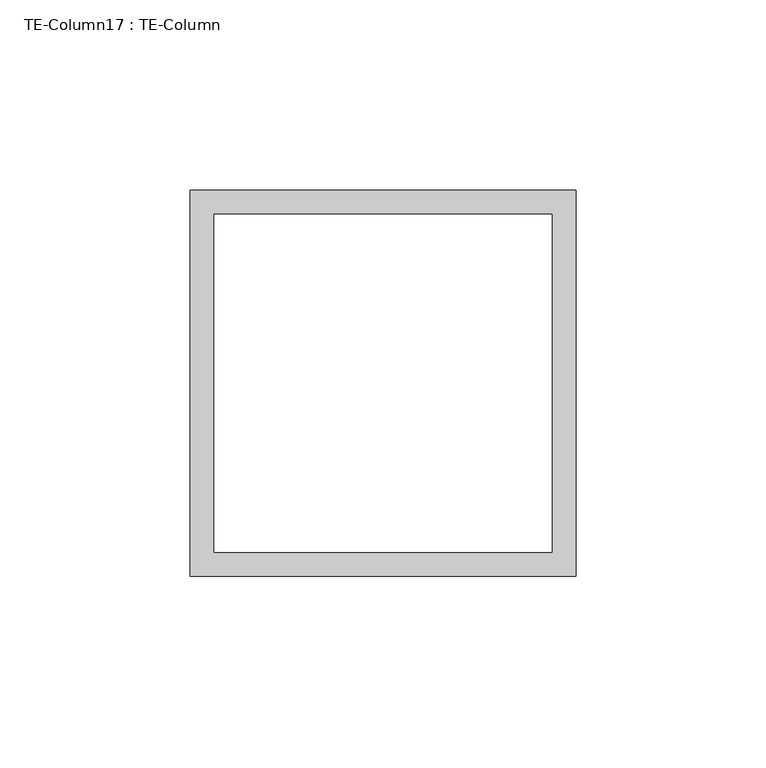
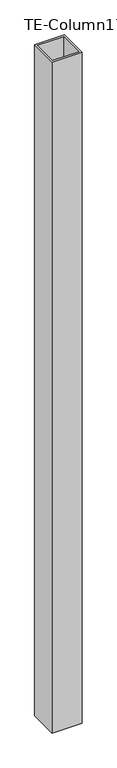
"""IFC4 building model written with IfcOpenShell, lengths in millimetres: proxy geometry, TE-Column17 : TE-Column."""

from ifc_helpers import new_model, si_unit, frame, origin, place, context, project, spatial, polyline, outline, extrude, source, transform, mapped, element, save


def te_column17_te_column_a47af242(model_context):
    return source(origin(), model_context, "Body", "SweptSolid", [
        extrude(outline(polyline([(590318.6434739, -536417.5913841), (590217.0434739, -536417.5913841), (590217.0434739, -536315.9913841), (590318.6434739, -536315.9913841), (590318.6434739, -536417.5913841)]), holes=[polyline([(590312.2934739, -536322.3413841), (590223.3934739, -536322.3413841), (590223.3934739, -536411.2413841), (590312.2934739, -536411.2413841), (590312.2934739, -536322.3413841)])]), frame((0.0, 0.0, 28.575), z_axis=(0.0, 0.0, 1.0), x_axis=(1.0, 0.0, 0.0)), (0.0, 0.0, 1.0), 2406.65),
    ])


if __name__ == "__main__":
    model = new_model("IFC4")
    model_context = context("Model", 3, world=origin())
    ifc_project = project(units=[si_unit("LENGTHUNIT", "METRE", prefix="MILLI")], contexts=[model_context])
    site = spatial("IfcSite", under=ifc_project)
    building = spatial("IfcBuilding", under=site)
    placement = place(None, origin())
    te_column17_te_column_shape = te_column17_te_column_a47af242(model_context)
    element("IfcBuildingElementProxy", 1, Name="TE-Column17 : TE-Column", ObjectType="TE-Column17 : TE-Column", at=placement, inside=building, context=model_context, shape_type="MappedRepresentation", body=[
        mapped(te_column17_te_column_shape, transform((0.0, 0.0, 0.0), x_axis=(1.0, 0.0, 0.0), y_axis=(0.0, 1.0, 0.0), z_axis=(0.0, 0.0, 1.0))),
    ])
    save(model, "model.ifc")

# Revit data of these elements
# Element 1 (IfcBuildingElementProxy, "TE-Column17 : TE-Column")
#   Materials on its faces: "4\"X4\" GALV. HSS TUBING"
# Materials
#   "4\"X4\" GALV. HSS TUBING": class "Generic", colour RGB 211 211 207, transparency 0, Cost = 0
